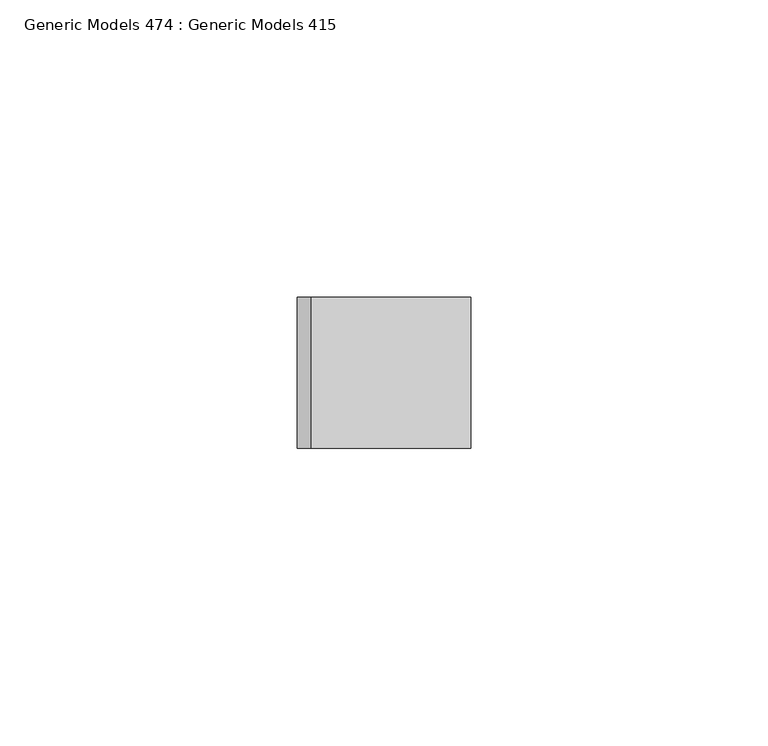
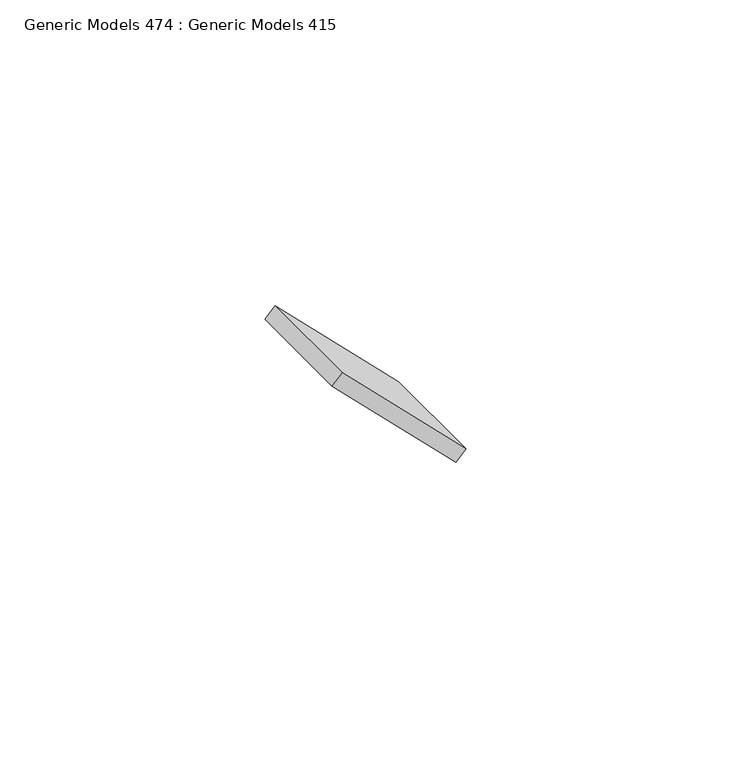
"""IFC4 building model written with IfcOpenShell, lengths in millimetres: proxy geometry, Generic Models 474 : Generic Models 415."""

from ifc_helpers import new_model, si_unit, frame, origin, place, context, project, spatial, polyline, outline, extrude, source, transform, mapped, element, save


def generic_models_474_generic_models_415_9ca26feb(model_context):
    return source(origin(), model_context, "Body", "SweptSolid", [
        extrude(outline(polyline([(0.0, -38.1), (0.0, 0.0), (25.4, 0.0), (25.4, -38.1), (0.0, -38.1)])), frame((-6869.8996186, -4475.9863946, 128035.5002957), z_axis=(0.7071067811864907, 0.0, 0.7071067811866044), x_axis=(0.0, -1.0, 0.0)), (0.0, 0.0, 1.0), 3.175),
    ])


if __name__ == "__main__":
    model = new_model("IFC4")
    model_context = context("Model", 3, world=origin())
    ifc_project = project(units=[si_unit("LENGTHUNIT", "METRE", prefix="MILLI")], contexts=[model_context])
    site = spatial("IfcSite", under=ifc_project)
    building = spatial("IfcBuilding", under=site)
    placement = place(None, origin())
    generic_models_474_generic_models_415_shape = generic_models_474_generic_models_415_9ca26feb(model_context)
    element("IfcBuildingElementProxy", 1, Name="Generic Models 474 : Generic Models 415", ObjectType="Generic Models 474 : Generic Models 415", at=placement, inside=building, context=model_context, shape_type="MappedRepresentation", body=[
        mapped(generic_models_474_generic_models_415_shape, transform((0.0, 0.0, 0.0), x_axis=(1.0, 0.0, 0.0), y_axis=(0.0, 1.0, 0.0), z_axis=(0.0, 0.0, 1.0))),
    ])
    save(model, "model.ifc")

# Revit data of these elements
# Element 1 (IfcBuildingElementProxy, "Generic Models 474 : Generic Models 415")
#   Materials on its faces: "_WELDED STEEL TABS FOR LOUVER ATTACHMENT"
# Materials
#   "_WELDED STEEL TABS FOR LOUVER ATTACHMENT": class "Metal", colour RGB 199 199 199, transparency 0, Description = "Structural steel 50ksi", Cost = 0
